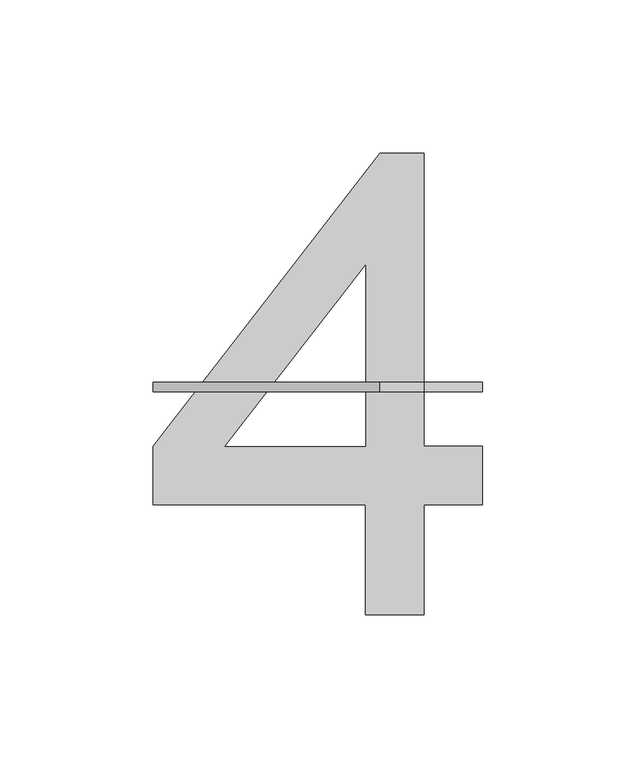
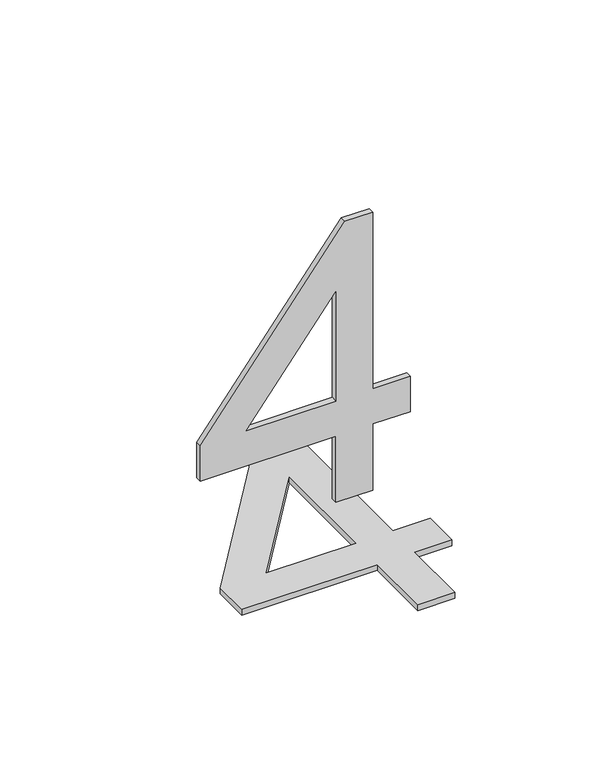
"""IFC4 building model written with IfcOpenShell, lengths in millimetres: proxy geometry, Grid Number1_FedEx : Grid Number1_FedEx."""

import ifcopenshell
import ifcopenshell.guid

model = None  # the IFC model being written
_history = None  # IfcOwnerHistory: only IFC2X3 demands one
_inside = {}  # id of a spatial element -> (the spatial element, [elements in it])
_under = {}  # id of a project, library or spatial element -> (it, [spatial elements below it])
_declared = {}  # id of a project -> (the project, [libraries it declares])
_typed = {}  # id of a type object -> (the type object, [elements of that type])
_made_of = {}  # id of a material, layer set ... -> (it, [elements and type objects made of it])


def new_model(schema):
    """Start an empty IFC model of exactly this schema.

    Asked for "IFC4X3", IfcOpenShell would pick the latest addendum, in which some entities
    have other attributes; the version numbers below select the first issue.
    IFC2X3 requires an IfcOwnerHistory on every rooted entity: one is made here for all.
    """
    global model, _history
    if schema == "IFC4X3":
        model = ifcopenshell.file(schema_version=(4, 3, 0, 0))
    else:
        model = ifcopenshell.file(schema=schema)
    _inside.clear()
    _under.clear()
    _declared.clear()
    _typed.clear()
    _made_of.clear()
    _history = None
    if model.schema == "IFC2X3":
        org = make("IfcOrganization", Name="unknown")
        user = make(
            "IfcPersonAndOrganization",
            ThePerson=make("IfcPerson", FamilyName="unknown"),
            TheOrganization=org,
        )
        app = make(
            "IfcApplication",
            ApplicationDeveloper=org,
            Version="unknown",
            ApplicationFullName="unknown",
            ApplicationIdentifier="unknown",
        )
        _history = make(
            "IfcOwnerHistory",
            OwningUser=user,
            OwningApplication=app,
            ChangeAction="ADDED",
            CreationDate=0,
        )
    return model


def make(cls, **values):
    """One entity of the class cls with the attributes given. An attribute that is None is left unset."""
    return model.create_entity(
        cls, **{name: value for name, value in values.items() if value is not None}
    )


def rooted(cls, **values):
    """An entity with a GlobalId (a new one), such as an element, a storey or a relation."""
    return make(cls, GlobalId=ifcopenshell.guid.new(), OwnerHistory=_history, **values)


def si_unit(unit_type, name, prefix=None):
    """IfcSIUnit, for example si_unit("LENGTHUNIT", "METRE", prefix="MILLI")."""
    return make("IfcSIUnit", UnitType=unit_type, Prefix=prefix, Name=name)


def assignment(units):
    """IfcUnitAssignment: the units of a project."""
    return None if units is None else make("IfcUnitAssignment", Units=units)


def point(xyz):
    """IfcCartesianPoint."""
    return None if xyz is None else make("IfcCartesianPoint", Coordinates=xyz)


def direction(xyz):
    """IfcDirection."""
    return None if xyz is None else make("IfcDirection", DirectionRatios=xyz)


def frame(location, z_axis=None, x_axis=None):
    """IfcAxis2Placement3D, a coordinate frame: its origin and axes. An axis left out is left unset."""
    return make(
        "IfcAxis2Placement3D",
        Location=point(location),
        Axis=direction(z_axis),
        RefDirection=direction(x_axis),
    )


def origin():
    """The frame at (0, 0, 0) with its axes left unset."""
    return frame((0.0, 0.0, 0.0))


def origin_with_axes():
    """The frame at (0, 0, 0) with the z axis (0, 0, 1) and the x axis (1, 0, 0) written out."""
    return frame((0.0, 0.0, 0.0), z_axis=(0.0, 0.0, 1.0), x_axis=(1.0, 0.0, 0.0))


def place(relative_to, where):
    """IfcLocalPlacement: puts the frame where relative to a parent placement (None: the world)."""
    return make(
        "IfcLocalPlacement", PlacementRelTo=relative_to, RelativePlacement=where
    )


def context(
    kind, dimensions, precision=None, world=None, true_north=None, identifier=None
):
    """IfcGeometricRepresentationContext, for example the 3D "Model" context."""
    return make(
        "IfcGeometricRepresentationContext",
        ContextIdentifier=identifier,
        ContextType=kind,
        CoordinateSpaceDimension=dimensions,
        Precision=precision,
        WorldCoordinateSystem=world,
        TrueNorth=true_north,
    )


def project(units=None, contexts=None):
    """IfcProject with its units and contexts."""
    return rooted(
        "IfcProject",
        Name="project",
        RepresentationContexts=contexts,
        UnitsInContext=assignment(units),
    )


def spatial(cls, under=None, at=None, **own):
    """A site, building, storey or space (cls), placed at a placement, below another one or the project."""
    s = rooted(cls, ObjectPlacement=at, **own)
    if under is not None:
        _under.setdefault(under.id(), (under, []))[1].append(s)
    return s


def polyline(points):
    """IfcPolyline through the points."""
    return make("IfcPolyline", Points=[point(p) for p in points])


def outline(outer, holes=None, kind="AREA"):
    """IfcArbitraryClosedProfileDef: a profile drawn as a closed curve; with holes, ...WithVoids."""
    if holes is None:
        return make("IfcArbitraryClosedProfileDef", ProfileType=kind, OuterCurve=outer)
    return make(
        "IfcArbitraryProfileDefWithVoids",
        ProfileType=kind,
        OuterCurve=outer,
        InnerCurves=holes,
    )


def extrude(swept, where, along, depth):
    """IfcExtrudedAreaSolid: the profile swept, set in the frame where, extruded along a direction by depth."""
    return make(
        "IfcExtrudedAreaSolid",
        SweptArea=swept,
        Position=where,
        ExtrudedDirection=direction(along),
        Depth=depth,
    )


def shape(context_of_items, identifier, shape_type, items):
    """IfcShapeRepresentation: the items that make up one representation, for example the "Body"."""
    return make(
        "IfcShapeRepresentation",
        ContextOfItems=context_of_items,
        RepresentationIdentifier=identifier,
        RepresentationType=shape_type,
        Items=items,
    )


def source(mapping_origin, context_of_items, identifier, shape_type, items):
    """IfcRepresentationMap: a shape defined once, which mapped items show again and again."""
    return make(
        "IfcRepresentationMap",
        MappingOrigin=mapping_origin,
        MappedRepresentation=shape(context_of_items, identifier, shape_type, items),
    )


def transform(
    local_origin,
    x_axis=None,
    y_axis=None,
    z_axis=None,
    scale=None,
    scale2=None,
    scale3=None,
    uniform=True,
):
    """IfcCartesianTransformationOperator3D, or its non-uniform kind. x_axis, y_axis, z_axis: its Axis1, 2, 3."""
    if uniform:
        return make(
            "IfcCartesianTransformationOperator3D",
            Axis1=direction(x_axis),
            Axis2=direction(y_axis),
            LocalOrigin=point(local_origin),
            Scale=scale,
            Axis3=direction(z_axis),
        )
    return make(
        "IfcCartesianTransformationOperator3DnonUniform",
        Axis1=direction(x_axis),
        Axis2=direction(y_axis),
        LocalOrigin=point(local_origin),
        Scale=scale,
        Axis3=direction(z_axis),
        Scale2=scale2,
        Scale3=scale3,
    )


def mapped(mapping_source, mapping_target):
    """IfcMappedItem: shows the shape of a source again, moved by a transform."""
    return make(
        "IfcMappedItem", MappingSource=mapping_source, MappingTarget=mapping_target
    )


def made_of(thing, what):
    """Note that an element or type object is made of a material, layer set ...; save() writes the relation."""
    if what is not None:
        _made_of.setdefault(what.id(), (what, []))[1].append(thing)
    return thing


def element(
    cls,
    number,
    at=None,
    inside=None,
    cuts=None,
    type_object=None,
    material=None,
    context=None,
    identifier="Body",
    shape_type=None,
    held_by="IfcProductDefinitionShape",
    body=None,
    shapes=None,
    **own,
):
    """One element of the class cls, such as IfcWall. Its Tag is "e" and its number.

    at: its placement. inside: the storey or other place that contains it. cuts: it is an
    opening in that element (IfcRelVoidsElement). A single representation is given by context,
    identifier, shape_type and body (its items); several are given by shapes. held_by: the class
    of the entity that holds the representations. save() writes the other relations.
    """
    e = rooted(cls, Tag="e%d" % number, ObjectPlacement=at, **own)
    if body is not None:
        shapes = [shape(context, identifier, shape_type, body)]
    if shapes is not None:
        e.Representation = make(held_by, Representations=shapes)
    if inside is not None:
        _inside.setdefault(inside.id(), (inside, []))[1].append(e)
    if cuts is not None:
        rooted(
            "IfcRelVoidsElement", RelatingBuildingElement=cuts, RelatedOpeningElement=e
        )
    if type_object is not None:
        _typed.setdefault(type_object.id(), (type_object, []))[1].append(e)
    return made_of(e, material)


def aggregate(whole, parts):
    """IfcRelAggregates: a whole, such as a stair, and the parts it consists of."""
    return rooted("IfcRelAggregates", RelatingObject=whole, RelatedObjects=parts)


def save(model, path):
    """Write the relations noted so far, then the file.

    IfcRelAggregates (storeys below a building ...), IfcRelContainedInSpatialStructure (elements
    in a storey), IfcRelDefinesByType, IfcRelAssociatesMaterial and IfcRelDeclares: one each for
    every whole, place, type object, material and project.
    """
    for whole, parts in _under.values():
        aggregate(whole, parts)
    for where, things in _inside.values():
        rooted(
            "IfcRelContainedInSpatialStructure",
            RelatedElements=things,
            RelatingStructure=where,
        )
    for kind, things in _typed.values():
        rooted("IfcRelDefinesByType", RelatedObjects=things, RelatingType=kind)
    for what, things in _made_of.values():
        rooted("IfcRelAssociatesMaterial", RelatedObjects=things, RelatingMaterial=what)
    for by, libraries in _declared.values():
        rooted("IfcRelDeclares", RelatingContext=by, RelatedDefinitions=libraries)
    model.write(path)


def entourage_2c91efbf(model_context):
    return source(origin(), model_context, "Body", "SweptSolid", [
        extrude(outline(polyline([(-94.9172894, 146.5840649), (-94.9172894, 182.4658032), (-164.28865, 182.4658032), (-164.28865, 201.6027303), (-90.1330576, 297.2873657), (-75.7803623, 297.2873657), (-75.7803623, 201.6027303), (-56.6434352, 201.6027303), (-56.6434352, 182.4658032), (-75.7803623, 182.4658032), (-75.7803623, 146.5840649), (-94.9172894, 146.5840649)]), holes=[polyline([(-94.9172894, 201.6027303), (-94.9172894, 260.7328448), (-140.7412593, 201.6027303), (-94.9172894, 201.6027303)])]), origin_with_axes(), (0.0, 0.0, 1.0), 3.175),
        extrude(outline(polyline([(14.4798932, -94.9172894), (14.4798932, -75.7803623), (50.3616315, -75.7803623), (50.3616315, -56.6434352), (69.4985586, -56.6434352), (69.4985586, -75.7803623), (165.183194, -75.7803623), (165.183194, -90.1330576), (69.4985586, -164.28865), (50.3616315, -164.28865), (50.3616315, -94.9172894), (14.4798932, -94.9172894)]), holes=[polyline([(69.4985586, -94.9172894), (69.4985586, -140.7412593), (128.6286732, -94.9172894), (69.4985586, -94.9172894)])]), frame((0.0, 219.3456765, 0.0), z_axis=(0.0, 1.0, 0.0), x_axis=(0.0, 0.0, 1.0)), (0.0, 0.0, 1.0), 3.175),
    ])


if __name__ == "__main__":
    model = new_model("IFC4")
    model_context = context("Model", 3, world=origin())
    ifc_project = project(units=[si_unit("LENGTHUNIT", "METRE", prefix="MILLI")], contexts=[model_context])
    site = spatial("IfcSite", under=ifc_project)
    building = spatial("IfcBuilding", under=site)
    placement = place(None, origin())
    entourage_shape = entourage_2c91efbf(model_context)
    element("IfcBuildingElementProxy", 1, Name="Grid Number1_FedEx : Grid Number1_FedEx", ObjectType="Grid Number1_FedEx : Grid Number1_FedEx", at=placement, inside=building, context=model_context, shape_type="MappedRepresentation", body=[
        mapped(entourage_shape, transform((0.0, 0.0, 0.0), x_axis=(1.0, 0.0, 0.0), y_axis=(0.0, 1.0, 0.0), z_axis=(0.0, 0.0, 1.0))),
    ])
    save(model, "model.ifc")

# Revit data of these elements
# Type "Grid Number1_FedEx : Grid Number1_FedEx"
#   Grid [instance default] = "S.8"
#   Label Width [instance default] = 1' - 0"
#   Half Box Width2 [instance default] = 0' - 6.13846"
#   Half Box Width [instance default] = 0' - 6"
#   Robust [instance default] = yes
#   Height = 0
#   Assembly Code = ""
# Element 1 (IfcBuildingElementProxy, "Grid Number1_FedEx : Grid Number1_FedEx")
#   Grid = "4"
#   Robust = no
#   Materials on its faces: "Letter"
# Materials
#   "Letter": class "Unassigned", colour RGB 178 187 30, transparency 0, Comments = "Rendering appearance not upgraded "
